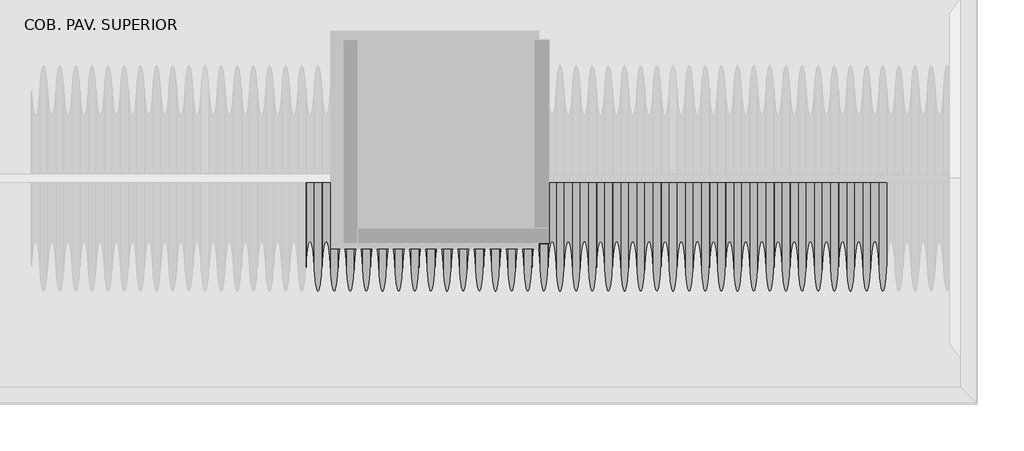
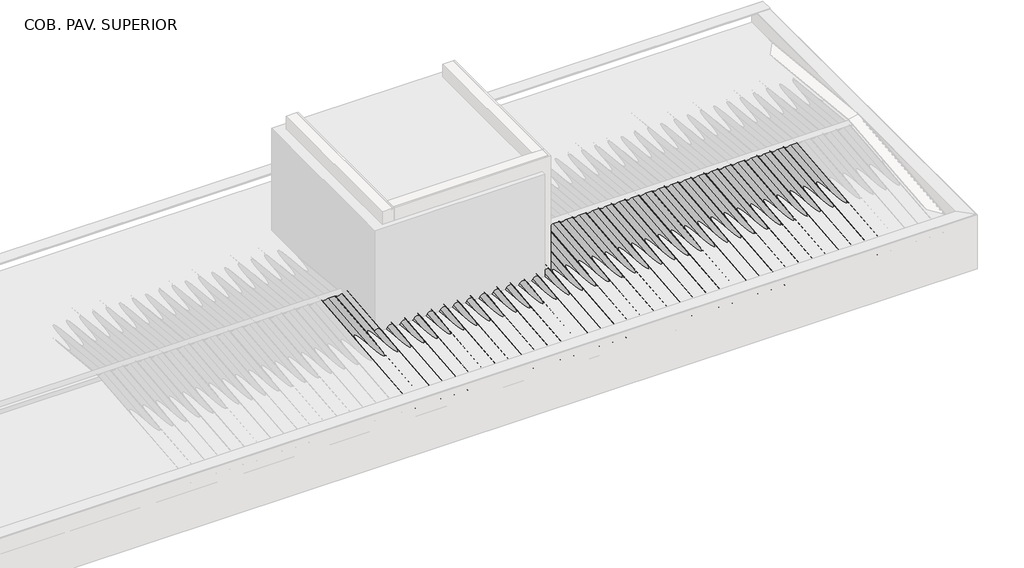
# One storey, part 6 of 8: 45 beams, 9 columns.
"""IFC4 building model written with IfcOpenShell, lengths in millimetres."""

import ifcopenshell
import ifcopenshell.guid

model = None  # the IFC model being written
_history = None  # IfcOwnerHistory: only IFC2X3 demands one
_inside = {}  # id of a spatial element -> (the spatial element, [elements in it])
_under = {}  # id of a project, library or spatial element -> (it, [spatial elements below it])
_declared = {}  # id of a project -> (the project, [libraries it declares])
_typed = {}  # id of a type object -> (the type object, [elements of that type])
_made_of = {}  # id of a material, layer set ... -> (it, [elements and type objects made of it])


def new_model(schema):
    """Start an empty IFC model of exactly this schema.

    Asked for "IFC4X3", IfcOpenShell would pick the latest addendum, in which some entities
    have other attributes; the version numbers below select the first issue.
    IFC2X3 requires an IfcOwnerHistory on every rooted entity: one is made here for all.
    """
    global model, _history
    if schema == "IFC4X3":
        model = ifcopenshell.file(schema_version=(4, 3, 0, 0))
    else:
        model = ifcopenshell.file(schema=schema)
    _inside.clear()
    _under.clear()
    _declared.clear()
    _typed.clear()
    _made_of.clear()
    _history = None
    if model.schema == "IFC2X3":
        org = make("IfcOrganization", Name="unknown")
        user = make(
            "IfcPersonAndOrganization",
            ThePerson=make("IfcPerson", FamilyName="unknown"),
            TheOrganization=org,
        )
        app = make(
            "IfcApplication",
            ApplicationDeveloper=org,
            Version="unknown",
            ApplicationFullName="unknown",
            ApplicationIdentifier="unknown",
        )
        _history = make(
            "IfcOwnerHistory",
            OwningUser=user,
            OwningApplication=app,
            ChangeAction="ADDED",
            CreationDate=0,
        )
    return model


def make(cls, **values):
    """One entity of the class cls with the attributes given. An attribute that is None is left unset."""
    return model.create_entity(
        cls, **{name: value for name, value in values.items() if value is not None}
    )


def rooted(cls, **values):
    """An entity with a GlobalId (a new one), such as an element, a storey or a relation."""
    return make(cls, GlobalId=ifcopenshell.guid.new(), OwnerHistory=_history, **values)


def si_unit(unit_type, name, prefix=None):
    """IfcSIUnit, for example si_unit("LENGTHUNIT", "METRE", prefix="MILLI")."""
    return make("IfcSIUnit", UnitType=unit_type, Prefix=prefix, Name=name)


def assignment(units):
    """IfcUnitAssignment: the units of a project."""
    return None if units is None else make("IfcUnitAssignment", Units=units)


def point(xyz):
    """IfcCartesianPoint."""
    return None if xyz is None else make("IfcCartesianPoint", Coordinates=xyz)


def direction(xyz):
    """IfcDirection."""
    return None if xyz is None else make("IfcDirection", DirectionRatios=xyz)


def frame(location, z_axis=None, x_axis=None):
    """IfcAxis2Placement3D, a coordinate frame: its origin and axes. An axis left out is left unset."""
    return make(
        "IfcAxis2Placement3D",
        Location=point(location),
        Axis=direction(z_axis),
        RefDirection=direction(x_axis),
    )


def frame_2d(location, x_axis=None):
    """IfcAxis2Placement2D, a coordinate frame in the plane: its origin and x axis."""
    return make(
        "IfcAxis2Placement2D", Location=point(location), RefDirection=direction(x_axis)
    )


def origin():
    """The frame at (0, 0, 0) with its axes left unset."""
    return frame((0.0, 0.0, 0.0))


def place(relative_to, where):
    """IfcLocalPlacement: puts the frame where relative to a parent placement (None: the world)."""
    return make(
        "IfcLocalPlacement", PlacementRelTo=relative_to, RelativePlacement=where
    )


def context(
    kind, dimensions, precision=None, world=None, true_north=None, identifier=None
):
    """IfcGeometricRepresentationContext, for example the 3D "Model" context."""
    return make(
        "IfcGeometricRepresentationContext",
        ContextIdentifier=identifier,
        ContextType=kind,
        CoordinateSpaceDimension=dimensions,
        Precision=precision,
        WorldCoordinateSystem=world,
        TrueNorth=true_north,
    )


def project(units=None, contexts=None):
    """IfcProject with its units and contexts."""
    return rooted(
        "IfcProject",
        Name="project",
        RepresentationContexts=contexts,
        UnitsInContext=assignment(units),
    )


def spatial(cls, under=None, at=None, **own):
    """A site, building, storey or space (cls), placed at a placement, below another one or the project."""
    s = rooted(cls, ObjectPlacement=at, **own)
    if under is not None:
        _under.setdefault(under.id(), (under, []))[1].append(s)
    return s


def polyline(points):
    """IfcPolyline through the points."""
    return make("IfcPolyline", Points=[point(p) for p in points])


def circle_curve(where, radius):
    """IfcCircle in the frame where."""
    return make("IfcCircle", Position=where, Radius=radius)


def trimmed(basis, trim1, trim2, sense, master):
    """IfcTrimmedCurve: the piece of a basis curve between two trims."""
    return make(
        "IfcTrimmedCurve",
        BasisCurve=basis,
        Trim1=trim1,
        Trim2=trim2,
        SenseAgreement=sense,
        MasterRepresentation=master,
    )


def segment(curve, same_sense, transition):
    """IfcCompositeCurveSegment."""
    return make(
        "IfcCompositeCurveSegment",
        Transition=transition,
        SameSense=same_sense,
        ParentCurve=curve,
    )


def composite_curve(segments, self_intersect=None):
    """IfcCompositeCurve: segments joined end to end."""
    return make("IfcCompositeCurve", Segments=segments, SelfIntersect=self_intersect)


def outline(outer, holes=None, kind="AREA"):
    """IfcArbitraryClosedProfileDef: a profile drawn as a closed curve; with holes, ...WithVoids."""
    if holes is None:
        return make("IfcArbitraryClosedProfileDef", ProfileType=kind, OuterCurve=outer)
    return make(
        "IfcArbitraryProfileDefWithVoids",
        ProfileType=kind,
        OuterCurve=outer,
        InnerCurves=holes,
    )


def extrude(swept, where, along, depth):
    """IfcExtrudedAreaSolid: the profile swept, set in the frame where, extruded along a direction by depth."""
    return make(
        "IfcExtrudedAreaSolid",
        SweptArea=swept,
        Position=where,
        ExtrudedDirection=direction(along),
        Depth=depth,
    )


def shape(context_of_items, identifier, shape_type, items):
    """IfcShapeRepresentation: the items that make up one representation, for example the "Body"."""
    return make(
        "IfcShapeRepresentation",
        ContextOfItems=context_of_items,
        RepresentationIdentifier=identifier,
        RepresentationType=shape_type,
        Items=items,
    )


def source(mapping_origin, context_of_items, identifier, shape_type, items):
    """IfcRepresentationMap: a shape defined once, which mapped items show again and again."""
    return make(
        "IfcRepresentationMap",
        MappingOrigin=mapping_origin,
        MappedRepresentation=shape(context_of_items, identifier, shape_type, items),
    )


def transform(
    local_origin,
    x_axis=None,
    y_axis=None,
    z_axis=None,
    scale=None,
    scale2=None,
    scale3=None,
    uniform=True,
):
    """IfcCartesianTransformationOperator3D, or its non-uniform kind. x_axis, y_axis, z_axis: its Axis1, 2, 3."""
    if uniform:
        return make(
            "IfcCartesianTransformationOperator3D",
            Axis1=direction(x_axis),
            Axis2=direction(y_axis),
            LocalOrigin=point(local_origin),
            Scale=scale,
            Axis3=direction(z_axis),
        )
    return make(
        "IfcCartesianTransformationOperator3DnonUniform",
        Axis1=direction(x_axis),
        Axis2=direction(y_axis),
        LocalOrigin=point(local_origin),
        Scale=scale,
        Axis3=direction(z_axis),
        Scale2=scale2,
        Scale3=scale3,
    )


def mapped(mapping_source, mapping_target):
    """IfcMappedItem: shows the shape of a source again, moved by a transform."""
    return make(
        "IfcMappedItem", MappingSource=mapping_source, MappingTarget=mapping_target
    )


def made_of(thing, what):
    """Note that an element or type object is made of a material, layer set ...; save() writes the relation."""
    if what is not None:
        _made_of.setdefault(what.id(), (what, []))[1].append(thing)
    return thing


def element(
    cls,
    number,
    at=None,
    inside=None,
    cuts=None,
    type_object=None,
    material=None,
    context=None,
    identifier="Body",
    shape_type=None,
    held_by="IfcProductDefinitionShape",
    body=None,
    shapes=None,
    **own,
):
    """One element of the class cls, such as IfcWall. Its Tag is "e" and its number.

    at: its placement. inside: the storey or other place that contains it. cuts: it is an
    opening in that element (IfcRelVoidsElement). A single representation is given by context,
    identifier, shape_type and body (its items); several are given by shapes. held_by: the class
    of the entity that holds the representations. save() writes the other relations.
    """
    e = rooted(cls, Tag="e%d" % number, ObjectPlacement=at, **own)
    if body is not None:
        shapes = [shape(context, identifier, shape_type, body)]
    if shapes is not None:
        e.Representation = make(held_by, Representations=shapes)
    if inside is not None:
        _inside.setdefault(inside.id(), (inside, []))[1].append(e)
    if cuts is not None:
        rooted(
            "IfcRelVoidsElement", RelatingBuildingElement=cuts, RelatedOpeningElement=e
        )
    if type_object is not None:
        _typed.setdefault(type_object.id(), (type_object, []))[1].append(e)
    return made_of(e, material)


def aggregate(whole, parts):
    """IfcRelAggregates: a whole, such as a stair, and the parts it consists of."""
    return rooted("IfcRelAggregates", RelatingObject=whole, RelatedObjects=parts)


def save(model, path):
    """Write the relations noted so far, then the file.

    IfcRelAggregates (storeys below a building ...), IfcRelContainedInSpatialStructure (elements
    in a storey), IfcRelDefinesByType, IfcRelAssociatesMaterial and IfcRelDeclares: one each for
    every whole, place, type object, material and project.
    """
    for whole, parts in _under.values():
        aggregate(whole, parts)
    for where, things in _inside.values():
        rooted(
            "IfcRelContainedInSpatialStructure",
            RelatedElements=things,
            RelatingStructure=where,
        )
    for kind, things in _typed.values():
        rooted("IfcRelDefinesByType", RelatedObjects=things, RelatingType=kind)
    for what, things in _made_of.values():
        rooted("IfcRelAssociatesMaterial", RelatedObjects=things, RelatingMaterial=what)
    for by, libraries in _declared.values():
        rooted("IfcRelDeclares", RelatingContext=by, RelatedDefinitions=libraries)
    model.write(path)


def beam_fe4ddbad(model_context):
    return source(origin(), model_context, "Body", "SweptSolid", [
        extrude(outline(polyline([(998.8971968, 30.0), (998.8971968, -30.0), (-998.8971974, -30.0), (-998.8971974, 30.0), (998.8971968, 30.0)])), frame((0.0, 0.0, -60.0), z_axis=(0.0, 0.0, 1.0), x_axis=(1.0, 0.0, 0.0)), (0.0, 0.0, 1.0), 120.0),
    ])


def beam_c6e4bd39(model_context):
    return source(origin(), model_context, "Body", "SweptSolid", [
        extrude(outline(polyline([(789.5373463, 30.0), (789.5373463, -30.0), (-789.5373463, -30.0), (-789.5373463, 30.0), (789.5373463, 30.0)])), frame((0.0, 0.0, -60.0), z_axis=(0.0, 0.0, 1.0), x_axis=(1.0, 0.0, 0.0)), (0.0, 0.0, 1.0), 120.0),
    ])


def telha_ondulada_fibrocimento_69359d52(model_context):
    return source(origin(), model_context, "Body", "SweptSolid", [
        extrude(outline(composite_curve([segment(trimmed(circle_curve(frame_2d((68.3970135, 71.7939461)), 66.7939461), [point((8.3970135, 42.4437972))], [point((128.3970135, 42.4437972))], True, "CARTESIAN"), True, "CONTINUOUS"), segment(polyline([(128.3970135, 42.4437972), (132.8884385, 40.2467307)]), True, "CONTINUOUS"), segment(trimmed(circle_curve(frame_2d((68.3970135, 71.7939461)), 71.7939461), [point((132.8884385, 40.2467307))], [point((3.9055884, 40.2467307))], False, "CARTESIAN"), True, "CONTINUOUS"), segment(trimmed(circle_curve(frame_2d((-51.6029865, 13.0936483)), 61.7939461), [point((3.9055884, 40.2467307))], [point((-107.1115615, 40.2467307))], True, "CARTESIAN"), True, "CONTINUOUS"), segment(polyline([(-107.1115615, 40.2467307), (-111.6029865, 42.4437972)]), True, "CONTINUOUS"), segment(trimmed(circle_curve(frame_2d((-51.6029865, 13.0936483)), 66.7939461), [point((-111.6029865, 42.4437972))], [point((8.3970135, 42.4437972))], False, "CARTESIAN"), True, "CONTINUOUS")], self_intersect=False)), frame((-1038.2805783, 0.0, 0.0), z_axis=(1.0, 0.0, 0.0), x_axis=(0.0, 1.0, 0.0)), (0.0, 0.0, 1.0), 2076.5611566),
    ])


def column_6c15bf79(model_context):
    return source(origin(), model_context, "Body", "SweptSolid", [
        extrude(outline(polyline([(30.0, 80.0), (30.0, -80.0), (-30.0, -80.0), (-30.0, 80.0), (30.0, 80.0)])), frame((0.0, 0.0, 6710.0), z_axis=(0.0, 0.0, 1.0), x_axis=(1.0, 0.0, 0.0)), (0.0, 0.0, 1.0), 467.5),
    ])


def column_42eef9f8(model_context):
    return source(origin(), model_context, "Body", "SweptSolid", [
        extrude(outline(polyline([(30.0, 80.0), (30.0, -80.0), (-30.0, -80.0), (-30.0, 80.0), (30.0, 80.0)])), frame((0.0, 0.0, 6710.0), z_axis=(0.0, 0.0, 1.0), x_axis=(1.0, 0.0, 0.0)), (0.0, 0.0, 1.0), 227.1),
    ])


model = new_model("IFC4")

# Units and contexts
model_context = context("Model", 3, world=origin())
ifc_project = project(units=[si_unit("LENGTHUNIT", "METRE", prefix="MILLI")], contexts=[model_context])

# Site, building, storey
site = spatial("IfcSite", under=ifc_project)
building = spatial("IfcBuilding", under=site)
storey = spatial("IfcBuildingStorey", under=building, Name="COB. PAV. SUPERIOR", Elevation=6650.0)

# Beams
placement = place(None, origin())
beam_shape = beam_fe4ddbad(model_context)
element("IfcBeam", 1, ObjectType="Madeira de lei : Berço 6x12cm", at=placement, inside=storey, context=model_context, shape_type="MappedRepresentation", body=[
    mapped(beam_shape, transform((248.5822594, -9189.768869, 6680.0), x_axis=(1.0, 0.0, 0.0), y_axis=(0.0, 0.0, -1.0), z_axis=(0.0, 1.0, 0.0))),
])
element("IfcBeam", 2, ObjectType="Madeira de lei : Berço 6x12cm", at=placement, inside=storey, context=model_context, shape_type="MappedRepresentation", body=[
    mapped(beam_shape, transform((2246.3766542, -9189.768869, 6680.0), x_axis=(1.0, 0.0, 0.0), y_axis=(0.0, 0.0, -1.0), z_axis=(0.0, 1.0, 0.0))),
])
element("IfcBeam", 3, ObjectType="Madeira de lei : Berço 6x12cm", at=placement, inside=storey, context=model_context, shape_type="MappedRepresentation", body=[
    mapped(beam_shape, transform((4244.171049, -9189.768869, 6680.0), x_axis=(1.0, 0.0, 0.0), y_axis=(0.0, 0.0, -1.0), z_axis=(0.0, 1.0, 0.0))),
])
element("IfcBeam", 4, ObjectType="Madeira de lei : Berço 6x12cm", at=placement, inside=storey, context=model_context, shape_type="MappedRepresentation", body=[
    mapped(beam_shape, transform((6241.9654438, -9189.768869, 6680.0), x_axis=(1.0, 0.0, 0.0), y_axis=(0.0, 0.0, -1.0), z_axis=(0.0, 1.0, 0.0))),
])
element("IfcBeam", 5, ObjectType="Madeira de lei : Berço 6x12cm", at=placement, inside=storey, context=model_context, shape_type="MappedRepresentation", body=[
    mapped(beam_shape, transform((8239.7598386, -9189.768869, 6680.0), x_axis=(1.0, 0.0, 0.0), y_axis=(0.0, 0.0, -1.0), z_axis=(0.0, 1.0, 0.0))),
])
element("IfcBeam", 6, ObjectType="Madeira de lei : Berço 6x12cm", at=placement, inside=storey, context=model_context, shape_type="MappedRepresentation", body=[
    mapped(beam_shape, transform((4244.171049, -10631.818869, 6680.0), x_axis=(1.0, 0.0, 0.0), y_axis=(0.0, 0.0, -1.0), z_axis=(0.0, 1.0, 0.0))),
])
element("IfcBeam", 7, ObjectType="Madeira de lei : Berço 6x12cm", at=placement, inside=storey, context=model_context, shape_type="MappedRepresentation", body=[
    mapped(beam_shape, transform((6241.9654438, -10631.818869, 6680.0), x_axis=(1.0, 0.0, 0.0), y_axis=(0.0, 0.0, -1.0), z_axis=(0.0, 1.0, 0.0))),
])
element("IfcBeam", 8, ObjectType="Madeira de lei : Berço 6x12cm", at=placement, inside=storey, context=model_context, shape_type="MappedRepresentation", body=[
    mapped(beam_shape, transform((8239.7598386, -10631.818869, 6680.0), x_axis=(1.0, 0.0, 0.0), y_axis=(0.0, 0.0, -1.0), z_axis=(0.0, 1.0, 0.0))),
])
beam_2_shape = beam_c6e4bd39(model_context)
element("IfcBeam", 9, ObjectType="Madeira de lei : Berço 6x12cm", at=placement, inside=storey, context=model_context, shape_type="MappedRepresentation", body=[
    mapped(beam_2_shape, transform((10028.1943824, -10631.818869, 6680.0), x_axis=(1.0, 0.0, 0.0), y_axis=(0.0, 0.0, -1.0), z_axis=(0.0, 1.0, 0.0))),
])
element("IfcBeam", 10, ObjectType="Telha Ondulada : Fibrocimento", at=placement, inside=storey, context=model_context, shape_type="SweptSolid", body=[
    extrude(outline(composite_curve([segment(trimmed(circle_curve(frame_2d((0.0, 66.7939461)), 66.7939461), [point((29.3501489, 6.7939461))], [point((29.3501489, 126.7939461))], True, "CARTESIAN"), True, "CONTINUOUS"), segment(polyline([(29.3501489, 126.7939461), (31.5472154, 131.2853711)]), True, "CONTINUOUS"), segment(trimmed(circle_curve(frame_2d((0.0, 66.7939461)), 71.7939461), [point((31.5472154, 131.2853711))], [point((31.5472154, 2.3025211))], False, "CARTESIAN"), True, "CONTINUOUS"), segment(trimmed(circle_curve(frame_2d((58.7002978, -53.2060539)), 61.7939461), [point((31.5472154, 2.3025211))], [point((31.5472154, -108.7146289))], True, "CARTESIAN"), True, "CONTINUOUS"), segment(polyline([(31.5472154, -108.7146289), (29.3501489, -113.2060539)]), True, "CONTINUOUS"), segment(trimmed(circle_curve(frame_2d((58.7002978, -53.2060539)), 66.7939461), [point((29.3501489, -113.2060539))], [point((29.3501489, 6.7939461))], False, "CARTESIAN"), True, "CONTINUOUS")], self_intersect=False)), frame((994.7156257, -10831.9594023, 7106.8215886), z_axis=(0.0, 0.9950371902099894, 0.09950371902099749), x_axis=(0.0, 0.09950371902099749, -0.9950371902099894)), (0.0, 0.0, 1.0), 3060.4439799),
])
element("IfcBeam", 11, ObjectType="Telha Ondulada : Fibrocimento", at=placement, inside=storey, context=model_context, shape_type="SweptSolid", body=[
    extrude(outline(composite_curve([segment(trimmed(circle_curve(frame_2d((0.0, 66.7939461)), 66.7939461), [point((29.3501489, 6.7939461))], [point((29.3501489, 126.7939461))], True, "CARTESIAN"), True, "CONTINUOUS"), segment(polyline([(29.3501489, 126.7939461), (31.5472154, 131.2853711)]), True, "CONTINUOUS"), segment(trimmed(circle_curve(frame_2d((0.0, 66.7939461)), 71.7939461), [point((31.5472154, 131.2853711))], [point((31.5472154, 2.3025211))], False, "CARTESIAN"), True, "CONTINUOUS"), segment(trimmed(circle_curve(frame_2d((58.7002978, -53.2060539)), 61.7939461), [point((31.5472154, 2.3025211))], [point((31.5472154, -108.7146289))], True, "CARTESIAN"), True, "CONTINUOUS"), segment(polyline([(31.5472154, -108.7146289), (29.3501489, -113.2060539)]), True, "CONTINUOUS"), segment(trimmed(circle_curve(frame_2d((58.7002978, -53.2060539)), 66.7939461), [point((29.3501489, -113.2060539))], [point((29.3501489, 6.7939461))], False, "CARTESIAN"), True, "CONTINUOUS")], self_intersect=False)), frame((1239.2156257, -10831.9594023, 7106.8215886), z_axis=(0.0, 0.9950371902099894, 0.09950371902099749), x_axis=(0.0, 0.09950371902099749, -0.9950371902099894)), (0.0, 0.0, 1.0), 3060.4439799),
])
element("IfcBeam", 12, ObjectType="Telha Ondulada : Fibrocimento", at=placement, inside=storey, context=model_context, shape_type="SweptSolid", body=[
    extrude(outline(composite_curve([segment(trimmed(circle_curve(frame_2d((0.0, 66.7939461)), 66.7939461), [point((29.3501489, 6.7939461))], [point((29.3501489, 126.7939461))], True, "CARTESIAN"), True, "CONTINUOUS"), segment(polyline([(29.3501489, 126.7939461), (31.5472154, 131.2853711)]), True, "CONTINUOUS"), segment(trimmed(circle_curve(frame_2d((0.0, 66.7939461)), 71.7939461), [point((31.5472154, 131.2853711))], [point((31.5472154, 2.3025211))], False, "CARTESIAN"), True, "CONTINUOUS"), segment(trimmed(circle_curve(frame_2d((58.7002978, -53.2060539)), 61.7939461), [point((31.5472154, 2.3025211))], [point((31.5472154, -108.7146289))], True, "CARTESIAN"), True, "CONTINUOUS"), segment(polyline([(31.5472154, -108.7146289), (29.3501489, -113.2060539)]), True, "CONTINUOUS"), segment(trimmed(circle_curve(frame_2d((58.7002978, -53.2060539)), 66.7939461), [point((29.3501489, -113.2060539))], [point((29.3501489, 6.7939461))], False, "CARTESIAN"), True, "CONTINUOUS")], self_intersect=False)), frame((4662.2156257, -10831.9594023, 7106.8215886), z_axis=(0.0, 0.9950371902099894, 0.09950371902099749), x_axis=(0.0, 0.09950371902099749, -0.9950371902099894)), (0.0, 0.0, 1.0), 3060.4439799),
])
element("IfcBeam", 13, ObjectType="Telha Ondulada : Fibrocimento", at=placement, inside=storey, context=model_context, shape_type="SweptSolid", body=[
    extrude(outline(composite_curve([segment(trimmed(circle_curve(frame_2d((0.0, 66.7939461)), 66.7939461), [point((29.3501489, 6.7939461))], [point((29.3501489, 126.7939461))], True, "CARTESIAN"), True, "CONTINUOUS"), segment(polyline([(29.3501489, 126.7939461), (31.5472154, 131.2853711)]), True, "CONTINUOUS"), segment(trimmed(circle_curve(frame_2d((0.0, 66.7939461)), 71.7939461), [point((31.5472154, 131.2853711))], [point((31.5472154, 2.3025211))], False, "CARTESIAN"), True, "CONTINUOUS"), segment(trimmed(circle_curve(frame_2d((58.7002978, -53.2060539)), 61.7939461), [point((31.5472154, 2.3025211))], [point((31.5472154, -108.7146289))], True, "CARTESIAN"), True, "CONTINUOUS"), segment(polyline([(31.5472154, -108.7146289), (29.3501489, -113.2060539)]), True, "CONTINUOUS"), segment(trimmed(circle_curve(frame_2d((58.7002978, -53.2060539)), 66.7939461), [point((29.3501489, -113.2060539))], [point((29.3501489, 6.7939461))], False, "CARTESIAN"), True, "CONTINUOUS")], self_intersect=False)), frame((4906.7156257, -10831.9594023, 7106.8215886), z_axis=(0.0, 0.9950371902099894, 0.09950371902099749), x_axis=(0.0, 0.09950371902099749, -0.9950371902099894)), (0.0, 0.0, 1.0), 3060.4439799),
])
element("IfcBeam", 14, ObjectType="Telha Ondulada : Fibrocimento", at=placement, inside=storey, context=model_context, shape_type="SweptSolid", body=[
    extrude(outline(composite_curve([segment(trimmed(circle_curve(frame_2d((0.0, 66.7939461)), 66.7939461), [point((29.3501489, 6.7939461))], [point((29.3501489, 126.7939461))], True, "CARTESIAN"), True, "CONTINUOUS"), segment(polyline([(29.3501489, 126.7939461), (31.5472154, 131.2853711)]), True, "CONTINUOUS"), segment(trimmed(circle_curve(frame_2d((0.0, 66.7939461)), 71.7939461), [point((31.5472154, 131.2853711))], [point((31.5472154, 2.3025211))], False, "CARTESIAN"), True, "CONTINUOUS"), segment(trimmed(circle_curve(frame_2d((58.7002978, -53.2060539)), 61.7939461), [point((31.5472154, 2.3025211))], [point((31.5472154, -108.7146289))], True, "CARTESIAN"), True, "CONTINUOUS"), segment(polyline([(31.5472154, -108.7146289), (29.3501489, -113.2060539)]), True, "CONTINUOUS"), segment(trimmed(circle_curve(frame_2d((58.7002978, -53.2060539)), 66.7939461), [point((29.3501489, -113.2060539))], [point((29.3501489, 6.7939461))], False, "CARTESIAN"), True, "CONTINUOUS")], self_intersect=False)), frame((5151.2156257, -10831.9594023, 7106.8215886), z_axis=(0.0, 0.9950371902099894, 0.09950371902099749), x_axis=(0.0, 0.09950371902099749, -0.9950371902099894)), (0.0, 0.0, 1.0), 3060.4439799),
])
element("IfcBeam", 15, ObjectType="Telha Ondulada : Fibrocimento", at=placement, inside=storey, context=model_context, shape_type="SweptSolid", body=[
    extrude(outline(composite_curve([segment(trimmed(circle_curve(frame_2d((0.0, 66.7939461)), 66.7939461), [point((29.3501489, 6.7939461))], [point((29.3501489, 126.7939461))], True, "CARTESIAN"), True, "CONTINUOUS"), segment(polyline([(29.3501489, 126.7939461), (31.5472154, 131.2853711)]), True, "CONTINUOUS"), segment(trimmed(circle_curve(frame_2d((0.0, 66.7939461)), 71.7939461), [point((31.5472154, 131.2853711))], [point((31.5472154, 2.3025211))], False, "CARTESIAN"), True, "CONTINUOUS"), segment(trimmed(circle_curve(frame_2d((58.7002978, -53.2060539)), 61.7939461), [point((31.5472154, 2.3025211))], [point((31.5472154, -108.7146289))], True, "CARTESIAN"), True, "CONTINUOUS"), segment(polyline([(31.5472154, -108.7146289), (29.3501489, -113.2060539)]), True, "CONTINUOUS"), segment(trimmed(circle_curve(frame_2d((58.7002978, -53.2060539)), 66.7939461), [point((29.3501489, -113.2060539))], [point((29.3501489, 6.7939461))], False, "CARTESIAN"), True, "CONTINUOUS")], self_intersect=False)), frame((5395.7156257, -10831.9594023, 7106.8215886), z_axis=(0.0, 0.9950371902099894, 0.09950371902099749), x_axis=(0.0, 0.09950371902099749, -0.9950371902099894)), (0.0, 0.0, 1.0), 3060.4439799),
])
element("IfcBeam", 16, ObjectType="Telha Ondulada : Fibrocimento", at=placement, inside=storey, context=model_context, shape_type="SweptSolid", body=[
    extrude(outline(composite_curve([segment(trimmed(circle_curve(frame_2d((0.0, 66.7939461)), 66.7939461), [point((29.3501489, 6.7939461))], [point((29.3501489, 126.7939461))], True, "CARTESIAN"), True, "CONTINUOUS"), segment(polyline([(29.3501489, 126.7939461), (31.5472154, 131.2853711)]), True, "CONTINUOUS"), segment(trimmed(circle_curve(frame_2d((0.0, 66.7939461)), 71.7939461), [point((31.5472154, 131.2853711))], [point((31.5472154, 2.3025211))], False, "CARTESIAN"), True, "CONTINUOUS"), segment(trimmed(circle_curve(frame_2d((58.7002978, -53.2060539)), 61.7939461), [point((31.5472154, 2.3025211))], [point((31.5472154, -108.7146289))], True, "CARTESIAN"), True, "CONTINUOUS"), segment(polyline([(31.5472154, -108.7146289), (29.3501489, -113.2060539)]), True, "CONTINUOUS"), segment(trimmed(circle_curve(frame_2d((58.7002978, -53.2060539)), 66.7939461), [point((29.3501489, -113.2060539))], [point((29.3501489, 6.7939461))], False, "CARTESIAN"), True, "CONTINUOUS")], self_intersect=False)), frame((5640.2156257, -10831.9594023, 7106.8215886), z_axis=(0.0, 0.9950371902099894, 0.09950371902099749), x_axis=(0.0, 0.09950371902099749, -0.9950371902099894)), (0.0, 0.0, 1.0), 3060.4439799),
])
element("IfcBeam", 17, ObjectType="Telha Ondulada : Fibrocimento", at=placement, inside=storey, context=model_context, shape_type="SweptSolid", body=[
    extrude(outline(composite_curve([segment(trimmed(circle_curve(frame_2d((0.0, 66.7939461)), 66.7939461), [point((29.3501489, 6.7939461))], [point((29.3501489, 126.7939461))], True, "CARTESIAN"), True, "CONTINUOUS"), segment(polyline([(29.3501489, 126.7939461), (31.5472154, 131.2853711)]), True, "CONTINUOUS"), segment(trimmed(circle_curve(frame_2d((0.0, 66.7939461)), 71.7939461), [point((31.5472154, 131.2853711))], [point((31.5472154, 2.3025211))], False, "CARTESIAN"), True, "CONTINUOUS"), segment(trimmed(circle_curve(frame_2d((58.7002978, -53.2060539)), 61.7939461), [point((31.5472154, 2.3025211))], [point((31.5472154, -108.7146289))], True, "CARTESIAN"), True, "CONTINUOUS"), segment(polyline([(31.5472154, -108.7146289), (29.3501489, -113.2060539)]), True, "CONTINUOUS"), segment(trimmed(circle_curve(frame_2d((58.7002978, -53.2060539)), 66.7939461), [point((29.3501489, -113.2060539))], [point((29.3501489, 6.7939461))], False, "CARTESIAN"), True, "CONTINUOUS")], self_intersect=False)), frame((5884.7156257, -10831.9594023, 7106.8215886), z_axis=(0.0, 0.9950371902099894, 0.09950371902099749), x_axis=(0.0, 0.09950371902099749, -0.9950371902099894)), (0.0, 0.0, 1.0), 3060.4439799),
])
element("IfcBeam", 18, ObjectType="Telha Ondulada : Fibrocimento", at=placement, inside=storey, context=model_context, shape_type="SweptSolid", body=[
    extrude(outline(composite_curve([segment(trimmed(circle_curve(frame_2d((0.0, 66.7939461)), 66.7939461), [point((29.3501489, 6.7939461))], [point((29.3501489, 126.7939461))], True, "CARTESIAN"), True, "CONTINUOUS"), segment(polyline([(29.3501489, 126.7939461), (31.5472154, 131.2853711)]), True, "CONTINUOUS"), segment(trimmed(circle_curve(frame_2d((0.0, 66.7939461)), 71.7939461), [point((31.5472154, 131.2853711))], [point((31.5472154, 2.3025211))], False, "CARTESIAN"), True, "CONTINUOUS"), segment(trimmed(circle_curve(frame_2d((58.7002978, -53.2060539)), 61.7939461), [point((31.5472154, 2.3025211))], [point((31.5472154, -108.7146289))], True, "CARTESIAN"), True, "CONTINUOUS"), segment(polyline([(31.5472154, -108.7146289), (29.3501489, -113.2060539)]), True, "CONTINUOUS"), segment(trimmed(circle_curve(frame_2d((58.7002978, -53.2060539)), 66.7939461), [point((29.3501489, -113.2060539))], [point((29.3501489, 6.7939461))], False, "CARTESIAN"), True, "CONTINUOUS")], self_intersect=False)), frame((6129.2156257, -10831.9594023, 7106.8215886), z_axis=(0.0, 0.9950371902099894, 0.09950371902099749), x_axis=(0.0, 0.09950371902099749, -0.9950371902099894)), (0.0, 0.0, 1.0), 3060.4439799),
])
element("IfcBeam", 19, ObjectType="Telha Ondulada : Fibrocimento", at=placement, inside=storey, context=model_context, shape_type="SweptSolid", body=[
    extrude(outline(composite_curve([segment(trimmed(circle_curve(frame_2d((0.0, 66.7939461)), 66.7939461), [point((29.3501489, 6.7939461))], [point((29.3501489, 126.7939461))], True, "CARTESIAN"), True, "CONTINUOUS"), segment(polyline([(29.3501489, 126.7939461), (31.5472154, 131.2853711)]), True, "CONTINUOUS"), segment(trimmed(circle_curve(frame_2d((0.0, 66.7939461)), 71.7939461), [point((31.5472154, 131.2853711))], [point((31.5472154, 2.3025211))], False, "CARTESIAN"), True, "CONTINUOUS"), segment(trimmed(circle_curve(frame_2d((58.7002978, -53.2060539)), 61.7939461), [point((31.5472154, 2.3025211))], [point((31.5472154, -108.7146289))], True, "CARTESIAN"), True, "CONTINUOUS"), segment(polyline([(31.5472154, -108.7146289), (29.3501489, -113.2060539)]), True, "CONTINUOUS"), segment(trimmed(circle_curve(frame_2d((58.7002978, -53.2060539)), 66.7939461), [point((29.3501489, -113.2060539))], [point((29.3501489, 6.7939461))], False, "CARTESIAN"), True, "CONTINUOUS")], self_intersect=False)), frame((6373.7156257, -10831.9594023, 7106.8215886), z_axis=(0.0, 0.9950371902099894, 0.09950371902099749), x_axis=(0.0, 0.09950371902099749, -0.9950371902099894)), (0.0, 0.0, 1.0), 3060.4439799),
])
element("IfcBeam", 20, ObjectType="Telha Ondulada : Fibrocimento", at=placement, inside=storey, context=model_context, shape_type="SweptSolid", body=[
    extrude(outline(composite_curve([segment(trimmed(circle_curve(frame_2d((0.0, 66.7939461)), 66.7939461), [point((29.3501489, 6.7939461))], [point((29.3501489, 126.7939461))], True, "CARTESIAN"), True, "CONTINUOUS"), segment(polyline([(29.3501489, 126.7939461), (31.5472154, 131.2853711)]), True, "CONTINUOUS"), segment(trimmed(circle_curve(frame_2d((0.0, 66.7939461)), 71.7939461), [point((31.5472154, 131.2853711))], [point((31.5472154, 2.3025211))], False, "CARTESIAN"), True, "CONTINUOUS"), segment(trimmed(circle_curve(frame_2d((58.7002978, -53.2060539)), 61.7939461), [point((31.5472154, 2.3025211))], [point((31.5472154, -108.7146289))], True, "CARTESIAN"), True, "CONTINUOUS"), segment(polyline([(31.5472154, -108.7146289), (29.3501489, -113.2060539)]), True, "CONTINUOUS"), segment(trimmed(circle_curve(frame_2d((58.7002978, -53.2060539)), 66.7939461), [point((29.3501489, -113.2060539))], [point((29.3501489, 6.7939461))], False, "CARTESIAN"), True, "CONTINUOUS")], self_intersect=False)), frame((6618.2156257, -10831.9594023, 7106.8215886), z_axis=(0.0, 0.9950371902099894, 0.09950371902099749), x_axis=(0.0, 0.09950371902099749, -0.9950371902099894)), (0.0, 0.0, 1.0), 3060.4439799),
])
element("IfcBeam", 21, ObjectType="Telha Ondulada : Fibrocimento", at=placement, inside=storey, context=model_context, shape_type="SweptSolid", body=[
    extrude(outline(composite_curve([segment(trimmed(circle_curve(frame_2d((0.0, 66.7939461)), 66.7939461), [point((29.3501489, 6.7939461))], [point((29.3501489, 126.7939461))], True, "CARTESIAN"), True, "CONTINUOUS"), segment(polyline([(29.3501489, 126.7939461), (31.5472154, 131.2853711)]), True, "CONTINUOUS"), segment(trimmed(circle_curve(frame_2d((0.0, 66.7939461)), 71.7939461), [point((31.5472154, 131.2853711))], [point((31.5472154, 2.3025211))], False, "CARTESIAN"), True, "CONTINUOUS"), segment(trimmed(circle_curve(frame_2d((58.7002978, -53.2060539)), 61.7939461), [point((31.5472154, 2.3025211))], [point((31.5472154, -108.7146289))], True, "CARTESIAN"), True, "CONTINUOUS"), segment(polyline([(31.5472154, -108.7146289), (29.3501489, -113.2060539)]), True, "CONTINUOUS"), segment(trimmed(circle_curve(frame_2d((58.7002978, -53.2060539)), 66.7939461), [point((29.3501489, -113.2060539))], [point((29.3501489, 6.7939461))], False, "CARTESIAN"), True, "CONTINUOUS")], self_intersect=False)), frame((6862.7156257, -10831.9594023, 7106.8215886), z_axis=(0.0, 0.9950371902099894, 0.09950371902099749), x_axis=(0.0, 0.09950371902099749, -0.9950371902099894)), (0.0, 0.0, 1.0), 3060.4439799),
])
element("IfcBeam", 22, ObjectType="Telha Ondulada : Fibrocimento", at=placement, inside=storey, context=model_context, shape_type="SweptSolid", body=[
    extrude(outline(composite_curve([segment(trimmed(circle_curve(frame_2d((0.0, 66.7939461)), 66.7939461), [point((29.3501489, 6.7939461))], [point((29.3501489, 126.7939461))], True, "CARTESIAN"), True, "CONTINUOUS"), segment(polyline([(29.3501489, 126.7939461), (31.5472154, 131.2853711)]), True, "CONTINUOUS"), segment(trimmed(circle_curve(frame_2d((0.0, 66.7939461)), 71.7939461), [point((31.5472154, 131.2853711))], [point((31.5472154, 2.3025211))], False, "CARTESIAN"), True, "CONTINUOUS"), segment(trimmed(circle_curve(frame_2d((58.7002978, -53.2060539)), 61.7939461), [point((31.5472154, 2.3025211))], [point((31.5472154, -108.7146289))], True, "CARTESIAN"), True, "CONTINUOUS"), segment(polyline([(31.5472154, -108.7146289), (29.3501489, -113.2060539)]), True, "CONTINUOUS"), segment(trimmed(circle_curve(frame_2d((58.7002978, -53.2060539)), 66.7939461), [point((29.3501489, -113.2060539))], [point((29.3501489, 6.7939461))], False, "CARTESIAN"), True, "CONTINUOUS")], self_intersect=False)), frame((7107.2156257, -10831.9594023, 7106.8215886), z_axis=(0.0, 0.9950371902099894, 0.09950371902099749), x_axis=(0.0, 0.09950371902099749, -0.9950371902099894)), (0.0, 0.0, 1.0), 3060.4439799),
])
element("IfcBeam", 23, ObjectType="Telha Ondulada : Fibrocimento", at=placement, inside=storey, context=model_context, shape_type="SweptSolid", body=[
    extrude(outline(composite_curve([segment(trimmed(circle_curve(frame_2d((0.0, 66.7939461)), 66.7939461), [point((29.3501489, 6.7939461))], [point((29.3501489, 126.7939461))], True, "CARTESIAN"), True, "CONTINUOUS"), segment(polyline([(29.3501489, 126.7939461), (31.5472154, 131.2853711)]), True, "CONTINUOUS"), segment(trimmed(circle_curve(frame_2d((0.0, 66.7939461)), 71.7939461), [point((31.5472154, 131.2853711))], [point((31.5472154, 2.3025211))], False, "CARTESIAN"), True, "CONTINUOUS"), segment(trimmed(circle_curve(frame_2d((58.7002978, -53.2060539)), 61.7939461), [point((31.5472154, 2.3025211))], [point((31.5472154, -108.7146289))], True, "CARTESIAN"), True, "CONTINUOUS"), segment(polyline([(31.5472154, -108.7146289), (29.3501489, -113.2060539)]), True, "CONTINUOUS"), segment(trimmed(circle_curve(frame_2d((58.7002978, -53.2060539)), 66.7939461), [point((29.3501489, -113.2060539))], [point((29.3501489, 6.7939461))], False, "CARTESIAN"), True, "CONTINUOUS")], self_intersect=False)), frame((7351.7156257, -10831.9594023, 7106.8215886), z_axis=(0.0, 0.9950371902099894, 0.09950371902099749), x_axis=(0.0, 0.09950371902099749, -0.9950371902099894)), (0.0, 0.0, 1.0), 3060.4439799),
])
element("IfcBeam", 24, ObjectType="Telha Ondulada : Fibrocimento", at=placement, inside=storey, context=model_context, shape_type="SweptSolid", body=[
    extrude(outline(composite_curve([segment(trimmed(circle_curve(frame_2d((0.0, 66.7939461)), 66.7939461), [point((29.3501489, 6.7939461))], [point((29.3501489, 126.7939461))], True, "CARTESIAN"), True, "CONTINUOUS"), segment(polyline([(29.3501489, 126.7939461), (31.5472154, 131.2853711)]), True, "CONTINUOUS"), segment(trimmed(circle_curve(frame_2d((0.0, 66.7939461)), 71.7939461), [point((31.5472154, 131.2853711))], [point((31.5472154, 2.3025211))], False, "CARTESIAN"), True, "CONTINUOUS"), segment(trimmed(circle_curve(frame_2d((58.7002978, -53.2060539)), 61.7939461), [point((31.5472154, 2.3025211))], [point((31.5472154, -108.7146289))], True, "CARTESIAN"), True, "CONTINUOUS"), segment(polyline([(31.5472154, -108.7146289), (29.3501489, -113.2060539)]), True, "CONTINUOUS"), segment(trimmed(circle_curve(frame_2d((58.7002978, -53.2060539)), 66.7939461), [point((29.3501489, -113.2060539))], [point((29.3501489, 6.7939461))], False, "CARTESIAN"), True, "CONTINUOUS")], self_intersect=False)), frame((7596.2156257, -10831.9594023, 7106.8215886), z_axis=(0.0, 0.9950371902099894, 0.09950371902099749), x_axis=(0.0, 0.09950371902099749, -0.9950371902099894)), (0.0, 0.0, 1.0), 3060.4439799),
])
element("IfcBeam", 25, ObjectType="Telha Ondulada : Fibrocimento", at=placement, inside=storey, context=model_context, shape_type="SweptSolid", body=[
    extrude(outline(composite_curve([segment(trimmed(circle_curve(frame_2d((0.0, 66.7939461)), 66.7939461), [point((29.3501489, 6.7939461))], [point((29.3501489, 126.7939461))], True, "CARTESIAN"), True, "CONTINUOUS"), segment(polyline([(29.3501489, 126.7939461), (31.5472154, 131.2853711)]), True, "CONTINUOUS"), segment(trimmed(circle_curve(frame_2d((0.0, 66.7939461)), 71.7939461), [point((31.5472154, 131.2853711))], [point((31.5472154, 2.3025211))], False, "CARTESIAN"), True, "CONTINUOUS"), segment(trimmed(circle_curve(frame_2d((58.7002978, -53.2060539)), 61.7939461), [point((31.5472154, 2.3025211))], [point((31.5472154, -108.7146289))], True, "CARTESIAN"), True, "CONTINUOUS"), segment(polyline([(31.5472154, -108.7146289), (29.3501489, -113.2060539)]), True, "CONTINUOUS"), segment(trimmed(circle_curve(frame_2d((58.7002978, -53.2060539)), 66.7939461), [point((29.3501489, -113.2060539))], [point((29.3501489, 6.7939461))], False, "CARTESIAN"), True, "CONTINUOUS")], self_intersect=False)), frame((7840.7156257, -10831.9594023, 7106.8215886), z_axis=(0.0, 0.9950371902099894, 0.09950371902099749), x_axis=(0.0, 0.09950371902099749, -0.9950371902099894)), (0.0, 0.0, 1.0), 3060.4439799),
])
element("IfcBeam", 26, ObjectType="Telha Ondulada : Fibrocimento", at=placement, inside=storey, context=model_context, shape_type="SweptSolid", body=[
    extrude(outline(composite_curve([segment(trimmed(circle_curve(frame_2d((0.0, 66.7939461)), 66.7939461), [point((29.3501489, 6.7939461))], [point((29.3501489, 126.7939461))], True, "CARTESIAN"), True, "CONTINUOUS"), segment(polyline([(29.3501489, 126.7939461), (31.5472154, 131.2853711)]), True, "CONTINUOUS"), segment(trimmed(circle_curve(frame_2d((0.0, 66.7939461)), 71.7939461), [point((31.5472154, 131.2853711))], [point((31.5472154, 2.3025211))], False, "CARTESIAN"), True, "CONTINUOUS"), segment(trimmed(circle_curve(frame_2d((58.7002978, -53.2060539)), 61.7939461), [point((31.5472154, 2.3025211))], [point((31.5472154, -108.7146289))], True, "CARTESIAN"), True, "CONTINUOUS"), segment(polyline([(31.5472154, -108.7146289), (29.3501489, -113.2060539)]), True, "CONTINUOUS"), segment(trimmed(circle_curve(frame_2d((58.7002978, -53.2060539)), 66.7939461), [point((29.3501489, -113.2060539))], [point((29.3501489, 6.7939461))], False, "CARTESIAN"), True, "CONTINUOUS")], self_intersect=False)), frame((8085.2156257, -10831.9594023, 7106.8215886), z_axis=(0.0, 0.9950371902099894, 0.09950371902099749), x_axis=(0.0, 0.09950371902099749, -0.9950371902099894)), (0.0, 0.0, 1.0), 3060.4439799),
])
element("IfcBeam", 27, ObjectType="Telha Ondulada : Fibrocimento", at=placement, inside=storey, context=model_context, shape_type="SweptSolid", body=[
    extrude(outline(composite_curve([segment(trimmed(circle_curve(frame_2d((0.0, 66.7939461)), 66.7939461), [point((29.3501489, 6.7939461))], [point((29.3501489, 126.7939461))], True, "CARTESIAN"), True, "CONTINUOUS"), segment(polyline([(29.3501489, 126.7939461), (31.5472154, 131.2853711)]), True, "CONTINUOUS"), segment(trimmed(circle_curve(frame_2d((0.0, 66.7939461)), 71.7939461), [point((31.5472154, 131.2853711))], [point((31.5472154, 2.3025211))], False, "CARTESIAN"), True, "CONTINUOUS"), segment(trimmed(circle_curve(frame_2d((58.7002978, -53.2060539)), 61.7939461), [point((31.5472154, 2.3025211))], [point((31.5472154, -108.7146289))], True, "CARTESIAN"), True, "CONTINUOUS"), segment(polyline([(31.5472154, -108.7146289), (29.3501489, -113.2060539)]), True, "CONTINUOUS"), segment(trimmed(circle_curve(frame_2d((58.7002978, -53.2060539)), 66.7939461), [point((29.3501489, -113.2060539))], [point((29.3501489, 6.7939461))], False, "CARTESIAN"), True, "CONTINUOUS")], self_intersect=False)), frame((8329.7156257, -10831.9594023, 7106.8215886), z_axis=(0.0, 0.9950371902099894, 0.09950371902099749), x_axis=(0.0, 0.09950371902099749, -0.9950371902099894)), (0.0, 0.0, 1.0), 3060.4439799),
])
element("IfcBeam", 28, ObjectType="Telha Ondulada : Fibrocimento", at=placement, inside=storey, context=model_context, shape_type="SweptSolid", body=[
    extrude(outline(composite_curve([segment(trimmed(circle_curve(frame_2d((0.0, 66.7939461)), 66.7939461), [point((29.3501489, 6.7939461))], [point((29.3501489, 126.7939461))], True, "CARTESIAN"), True, "CONTINUOUS"), segment(polyline([(29.3501489, 126.7939461), (31.5472154, 131.2853711)]), True, "CONTINUOUS"), segment(trimmed(circle_curve(frame_2d((0.0, 66.7939461)), 71.7939461), [point((31.5472154, 131.2853711))], [point((31.5472154, 2.3025211))], False, "CARTESIAN"), True, "CONTINUOUS"), segment(trimmed(circle_curve(frame_2d((58.7002978, -53.2060539)), 61.7939461), [point((31.5472154, 2.3025211))], [point((31.5472154, -108.7146289))], True, "CARTESIAN"), True, "CONTINUOUS"), segment(polyline([(31.5472154, -108.7146289), (29.3501489, -113.2060539)]), True, "CONTINUOUS"), segment(trimmed(circle_curve(frame_2d((58.7002978, -53.2060539)), 66.7939461), [point((29.3501489, -113.2060539))], [point((29.3501489, 6.7939461))], False, "CARTESIAN"), True, "CONTINUOUS")], self_intersect=False)), frame((8574.2156257, -10831.9594023, 7106.8215886), z_axis=(0.0, 0.9950371902099894, 0.09950371902099749), x_axis=(0.0, 0.09950371902099749, -0.9950371902099894)), (0.0, 0.0, 1.0), 3060.4439799),
])
element("IfcBeam", 29, ObjectType="Telha Ondulada : Fibrocimento", at=placement, inside=storey, context=model_context, shape_type="SweptSolid", body=[
    extrude(outline(composite_curve([segment(trimmed(circle_curve(frame_2d((0.0, 66.7939461)), 66.7939461), [point((29.3501489, 6.7939461))], [point((29.3501489, 126.7939461))], True, "CARTESIAN"), True, "CONTINUOUS"), segment(polyline([(29.3501489, 126.7939461), (31.5472154, 131.2853711)]), True, "CONTINUOUS"), segment(trimmed(circle_curve(frame_2d((0.0, 66.7939461)), 71.7939461), [point((31.5472154, 131.2853711))], [point((31.5472154, 2.3025211))], False, "CARTESIAN"), True, "CONTINUOUS"), segment(trimmed(circle_curve(frame_2d((58.7002978, -53.2060539)), 61.7939461), [point((31.5472154, 2.3025211))], [point((31.5472154, -108.7146289))], True, "CARTESIAN"), True, "CONTINUOUS"), segment(polyline([(31.5472154, -108.7146289), (29.3501489, -113.2060539)]), True, "CONTINUOUS"), segment(trimmed(circle_curve(frame_2d((58.7002978, -53.2060539)), 66.7939461), [point((29.3501489, -113.2060539))], [point((29.3501489, 6.7939461))], False, "CARTESIAN"), True, "CONTINUOUS")], self_intersect=False)), frame((8818.7156257, -10831.9594023, 7106.8215886), z_axis=(0.0, 0.9950371902099894, 0.09950371902099749), x_axis=(0.0, 0.09950371902099749, -0.9950371902099894)), (0.0, 0.0, 1.0), 3060.4439799),
])
element("IfcBeam", 30, ObjectType="Telha Ondulada : Fibrocimento", at=placement, inside=storey, context=model_context, shape_type="SweptSolid", body=[
    extrude(outline(composite_curve([segment(trimmed(circle_curve(frame_2d((0.0, 66.7939461)), 66.7939461), [point((29.3501489, 6.7939461))], [point((29.3501489, 126.7939461))], True, "CARTESIAN"), True, "CONTINUOUS"), segment(polyline([(29.3501489, 126.7939461), (31.5472154, 131.2853711)]), True, "CONTINUOUS"), segment(trimmed(circle_curve(frame_2d((0.0, 66.7939461)), 71.7939461), [point((31.5472154, 131.2853711))], [point((31.5472154, 2.3025211))], False, "CARTESIAN"), True, "CONTINUOUS"), segment(trimmed(circle_curve(frame_2d((58.7002978, -53.2060539)), 61.7939461), [point((31.5472154, 2.3025211))], [point((31.5472154, -108.7146289))], True, "CARTESIAN"), True, "CONTINUOUS"), segment(polyline([(31.5472154, -108.7146289), (29.3501489, -113.2060539)]), True, "CONTINUOUS"), segment(trimmed(circle_curve(frame_2d((58.7002978, -53.2060539)), 66.7939461), [point((29.3501489, -113.2060539))], [point((29.3501489, 6.7939461))], False, "CARTESIAN"), True, "CONTINUOUS")], self_intersect=False)), frame((9063.2156257, -10831.9594023, 7106.8215886), z_axis=(0.0, 0.9950371902099894, 0.09950371902099749), x_axis=(0.0, 0.09950371902099749, -0.9950371902099894)), (0.0, 0.0, 1.0), 3060.4439799),
])
element("IfcBeam", 31, ObjectType="Telha Ondulada : Fibrocimento", at=placement, inside=storey, context=model_context, shape_type="SweptSolid", body=[
    extrude(outline(composite_curve([segment(trimmed(circle_curve(frame_2d((0.0, 66.7939461)), 66.7939461), [point((29.3501489, 6.7939461))], [point((29.3501489, 126.7939461))], True, "CARTESIAN"), True, "CONTINUOUS"), segment(polyline([(29.3501489, 126.7939461), (31.5472154, 131.2853711)]), True, "CONTINUOUS"), segment(trimmed(circle_curve(frame_2d((0.0, 66.7939461)), 71.7939461), [point((31.5472154, 131.2853711))], [point((31.5472154, 2.3025211))], False, "CARTESIAN"), True, "CONTINUOUS"), segment(trimmed(circle_curve(frame_2d((58.7002978, -53.2060539)), 61.7939461), [point((31.5472154, 2.3025211))], [point((31.5472154, -108.7146289))], True, "CARTESIAN"), True, "CONTINUOUS"), segment(polyline([(31.5472154, -108.7146289), (29.3501489, -113.2060539)]), True, "CONTINUOUS"), segment(trimmed(circle_curve(frame_2d((58.7002978, -53.2060539)), 66.7939461), [point((29.3501489, -113.2060539))], [point((29.3501489, 6.7939461))], False, "CARTESIAN"), True, "CONTINUOUS")], self_intersect=False)), frame((9307.7156257, -10831.9594023, 7106.8215886), z_axis=(0.0, 0.9950371902099894, 0.09950371902099749), x_axis=(0.0, 0.09950371902099749, -0.9950371902099894)), (0.0, 0.0, 1.0), 3060.4439799),
])
element("IfcBeam", 32, ObjectType="Telha Ondulada : Fibrocimento", at=placement, inside=storey, context=model_context, shape_type="SweptSolid", body=[
    extrude(outline(composite_curve([segment(trimmed(circle_curve(frame_2d((0.0, 66.7939461)), 66.7939461), [point((29.3501489, 6.7939461))], [point((29.3501489, 126.7939461))], True, "CARTESIAN"), True, "CONTINUOUS"), segment(polyline([(29.3501489, 126.7939461), (31.5472154, 131.2853711)]), True, "CONTINUOUS"), segment(trimmed(circle_curve(frame_2d((0.0, 66.7939461)), 71.7939461), [point((31.5472154, 131.2853711))], [point((31.5472154, 2.3025211))], False, "CARTESIAN"), True, "CONTINUOUS"), segment(trimmed(circle_curve(frame_2d((58.7002978, -53.2060539)), 61.7939461), [point((31.5472154, 2.3025211))], [point((31.5472154, -108.7146289))], True, "CARTESIAN"), True, "CONTINUOUS"), segment(polyline([(31.5472154, -108.7146289), (29.3501489, -113.2060539)]), True, "CONTINUOUS"), segment(trimmed(circle_curve(frame_2d((58.7002978, -53.2060539)), 66.7939461), [point((29.3501489, -113.2060539))], [point((29.3501489, 6.7939461))], False, "CARTESIAN"), True, "CONTINUOUS")], self_intersect=False)), frame((9552.2156257, -10831.9594023, 7106.8215886), z_axis=(0.0, 0.9950371902099894, 0.09950371902099749), x_axis=(0.0, 0.09950371902099749, -0.9950371902099894)), (0.0, 0.0, 1.0), 3060.4439799),
])
telha_ondulada_fibrocimento_shape = telha_ondulada_fibrocimento_69359d52(model_context)
element("IfcBeam", 33, ObjectType="Telha Ondulada : Fibrocimento", at=placement, inside=storey, context=model_context, shape_type="MappedRepresentation", body=[
    mapped(telha_ondulada_fibrocimento_shape, transform((1485.318693, -9791.6878483, 7138.6967211), x_axis=(0.0, 0.9950371902099893, 0.09950371902099736), y_axis=(-1.0, 0.0, 0.0), z_axis=(0.0, -0.09950371902099737, 0.9950371902099894))),
])
element("IfcBeam", 34, ObjectType="Telha Ondulada : Fibrocimento", at=placement, inside=storey, context=model_context, shape_type="MappedRepresentation", body=[
    mapped(telha_ondulada_fibrocimento_shape, transform((1729.818693, -9791.6878483, 7138.6967211), x_axis=(0.0, 0.9950371902099893, 0.09950371902099736), y_axis=(-1.0, 0.0, 0.0), z_axis=(0.0, -0.09950371902099737, 0.9950371902099894))),
])
element("IfcBeam", 35, ObjectType="Telha Ondulada : Fibrocimento", at=placement, inside=storey, context=model_context, shape_type="MappedRepresentation", body=[
    mapped(telha_ondulada_fibrocimento_shape, transform((1974.318693, -9791.6878483, 7138.6967211), x_axis=(0.0, 0.9950371902099893, 0.09950371902099736), y_axis=(-1.0, 0.0, 0.0), z_axis=(0.0, -0.09950371902099737, 0.9950371902099894))),
])
element("IfcBeam", 36, ObjectType="Telha Ondulada : Fibrocimento", at=placement, inside=storey, context=model_context, shape_type="MappedRepresentation", body=[
    mapped(telha_ondulada_fibrocimento_shape, transform((2218.818693, -9791.6878483, 7138.6967211), x_axis=(0.0, 0.9950371902099893, 0.09950371902099736), y_axis=(-1.0, 0.0, 0.0), z_axis=(0.0, -0.09950371902099737, 0.9950371902099894))),
])
element("IfcBeam", 37, ObjectType="Telha Ondulada : Fibrocimento", at=placement, inside=storey, context=model_context, shape_type="MappedRepresentation", body=[
    mapped(telha_ondulada_fibrocimento_shape, transform((2463.318693, -9791.6878483, 7138.6967211), x_axis=(0.0, 0.9950371902099893, 0.09950371902099736), y_axis=(-1.0, 0.0, 0.0), z_axis=(0.0, -0.09950371902099737, 0.9950371902099894))),
])
element("IfcBeam", 38, ObjectType="Telha Ondulada : Fibrocimento", at=placement, inside=storey, context=model_context, shape_type="MappedRepresentation", body=[
    mapped(telha_ondulada_fibrocimento_shape, transform((2707.818693, -9791.6878483, 7138.6967211), x_axis=(0.0, 0.9950371902099893, 0.09950371902099736), y_axis=(-1.0, 0.0, 0.0), z_axis=(0.0, -0.09950371902099737, 0.9950371902099894))),
])
element("IfcBeam", 39, ObjectType="Telha Ondulada : Fibrocimento", at=placement, inside=storey, context=model_context, shape_type="MappedRepresentation", body=[
    mapped(telha_ondulada_fibrocimento_shape, transform((2952.318693, -9791.6878483, 7138.6967211), x_axis=(0.0, 0.9950371902099893, 0.09950371902099736), y_axis=(-1.0, 0.0, 0.0), z_axis=(0.0, -0.09950371902099737, 0.9950371902099894))),
])
element("IfcBeam", 40, ObjectType="Telha Ondulada : Fibrocimento", at=placement, inside=storey, context=model_context, shape_type="MappedRepresentation", body=[
    mapped(telha_ondulada_fibrocimento_shape, transform((3196.818693, -9791.6878483, 7138.6967211), x_axis=(0.0, 0.9950371902099893, 0.09950371902099736), y_axis=(-1.0, 0.0, 0.0), z_axis=(0.0, -0.09950371902099737, 0.9950371902099894))),
])
element("IfcBeam", 41, ObjectType="Telha Ondulada : Fibrocimento", at=placement, inside=storey, context=model_context, shape_type="MappedRepresentation", body=[
    mapped(telha_ondulada_fibrocimento_shape, transform((3441.318693, -9791.6878483, 7138.6967211), x_axis=(0.0, 0.9950371902099893, 0.09950371902099736), y_axis=(-1.0, 0.0, 0.0), z_axis=(0.0, -0.09950371902099737, 0.9950371902099894))),
])
element("IfcBeam", 42, ObjectType="Telha Ondulada : Fibrocimento", at=placement, inside=storey, context=model_context, shape_type="MappedRepresentation", body=[
    mapped(telha_ondulada_fibrocimento_shape, transform((3685.818693, -9791.6878483, 7138.6967211), x_axis=(0.0, 0.9950371902099893, 0.09950371902099736), y_axis=(-1.0, 0.0, 0.0), z_axis=(0.0, -0.09950371902099737, 0.9950371902099894))),
])
element("IfcBeam", 43, ObjectType="Telha Ondulada : Fibrocimento", at=placement, inside=storey, context=model_context, shape_type="MappedRepresentation", body=[
    mapped(telha_ondulada_fibrocimento_shape, transform((3930.318693, -9791.6878483, 7138.6967211), x_axis=(0.0, 0.9950371902099893, 0.09950371902099736), y_axis=(-1.0, 0.0, 0.0), z_axis=(0.0, -0.09950371902099737, 0.9950371902099894))),
])
element("IfcBeam", 44, ObjectType="Telha Ondulada : Fibrocimento", at=placement, inside=storey, context=model_context, shape_type="MappedRepresentation", body=[
    mapped(telha_ondulada_fibrocimento_shape, transform((4174.818693, -9791.6878483, 7138.6967211), x_axis=(0.0, 0.9950371902099893, 0.09950371902099736), y_axis=(-1.0, 0.0, 0.0), z_axis=(0.0, -0.09950371902099737, 0.9950371902099894))),
])
element("IfcBeam", 45, ObjectType="Telha Ondulada : Fibrocimento", at=placement, inside=storey, context=model_context, shape_type="MappedRepresentation", body=[
    mapped(telha_ondulada_fibrocimento_shape, transform((4419.318693, -9791.6878483, 7138.6967211), x_axis=(0.0, 0.9950371902099893, 0.09950371902099736), y_axis=(-1.0, 0.0, 0.0), z_axis=(0.0, -0.09950371902099737, 0.9950371902099894))),
])

# Columns
column_shape = column_6c15bf79(model_context)
element("IfcColumn", 46, ObjectType="Madeira de lei-Coluna : Pontalete 6X16cm", at=placement, inside=storey, context=model_context, shape_type="MappedRepresentation", body=[
    mapped(column_shape, transform((248.5822594, -9189.768869, 0.0), x_axis=(0.0, -1.0, 0.0), y_axis=(1.0, 0.0, 0.0), z_axis=(0.0, 0.0, 1.0))),
])
element("IfcColumn", 47, ObjectType="Madeira de lei-Coluna : Pontalete 6X16cm", at=placement, inside=storey, context=model_context, shape_type="MappedRepresentation", body=[
    mapped(column_shape, transform((2246.3766542, -9189.768869, 0.0), x_axis=(0.0, -1.0, 0.0), y_axis=(1.0, 0.0, 0.0), z_axis=(0.0, 0.0, 1.0))),
])
element("IfcColumn", 48, ObjectType="Madeira de lei-Coluna : Pontalete 6X16cm", at=placement, inside=storey, context=model_context, shape_type="MappedRepresentation", body=[
    mapped(column_shape, transform((4244.171049, -9189.768869, 0.0), x_axis=(0.0, -1.0, 0.0), y_axis=(1.0, 0.0, 0.0), z_axis=(0.0, 0.0, 1.0))),
])
element("IfcColumn", 49, ObjectType="Madeira de lei-Coluna : Pontalete 6X16cm", at=placement, inside=storey, context=model_context, shape_type="MappedRepresentation", body=[
    mapped(column_shape, transform((6241.9654438, -9189.768869, 0.0), x_axis=(0.0, -1.0, 0.0), y_axis=(1.0, 0.0, 0.0), z_axis=(0.0, 0.0, 1.0))),
])
element("IfcColumn", 50, ObjectType="Madeira de lei-Coluna : Pontalete 6X16cm", at=placement, inside=storey, context=model_context, shape_type="MappedRepresentation", body=[
    mapped(column_shape, transform((8239.7598386, -9189.768869, 0.0), x_axis=(0.0, -1.0, 0.0), y_axis=(1.0, 0.0, 0.0), z_axis=(0.0, 0.0, 1.0))),
])
column_2_shape = column_42eef9f8(model_context)
element("IfcColumn", 51, ObjectType="Madeira de lei-Coluna : Pontalete 6X16cm", at=placement, inside=storey, context=model_context, shape_type="MappedRepresentation", body=[
    mapped(column_2_shape, transform((4244.171049, -10631.818869, 0.0), x_axis=(0.0, -1.0, 0.0), y_axis=(1.0, 0.0, 0.0), z_axis=(0.0, 0.0, 1.0))),
])
element("IfcColumn", 52, ObjectType="Madeira de lei-Coluna : Pontalete 6X16cm", at=placement, inside=storey, context=model_context, shape_type="MappedRepresentation", body=[
    mapped(column_2_shape, transform((6241.9654438, -10631.818869, 0.0), x_axis=(0.0, -1.0, 0.0), y_axis=(1.0, 0.0, 0.0), z_axis=(0.0, 0.0, 1.0))),
])
element("IfcColumn", 53, ObjectType="Madeira de lei-Coluna : Pontalete 6X16cm", at=placement, inside=storey, context=model_context, shape_type="MappedRepresentation", body=[
    mapped(column_2_shape, transform((8239.7598386, -10631.818869, 0.0), x_axis=(0.0, -1.0, 0.0), y_axis=(1.0, 0.0, 0.0), z_axis=(0.0, 0.0, 1.0))),
])
element("IfcColumn", 54, ObjectType="Madeira de lei-Coluna : Pontalete 6X16cm", at=placement, inside=storey, context=model_context, shape_type="MappedRepresentation", body=[
    mapped(column_2_shape, transform((10237.5542335, -10631.818869, 0.0), x_axis=(0.0, -1.0, 0.0), y_axis=(1.0, 0.0, 0.0), z_axis=(0.0, 0.0, 1.0))),
])

save(model, "model.ifc")

# Revit data of these elements
# Type "Madeira de lei : Berço 6x12cm"
#   A = 0.02 m²
#   Length [instance default] = 1.524 m
#   b = 0.06 m
#   d = 0.12 m
#   Structural Material [instance default] = none
#   Assembly Code = ""
# Type "Telha Ondulada : Fibrocimento"
#   Description = "TELHA ONDULADA FIBROCIMENTO"
#   Cost = 5
#   Length [instance default] = 1.524 m
#   b = 0.07 m
#   h = 0.16 m
#   Structural Material = .TELHA DE FIBROCIMENTO
#   Assembly Code = ""
# Type "Madeira de lei-Coluna : Pontalete 6X16cm"
#   A = 0.01952 m²
#   b = 0.06 m
#   d = 0.16 m
#   Structural Material [instance default] = none
#   Assembly Code = ""
# Elements 1, 2, 3, 4, 5, 6, 7, 8 (IfcBeam, "Madeira de lei : Berço 6x12cm")
#   Comments = ""
#   Uso = "TELHADOS ESTRUTURAS"
#   Compr Cmcl = 6.00 m
#   Structural Material = .MADEIRAMENTO
#   Phase Created = CC_AP
#   Materials on its faces: ".MADEIRAMENTO"
# Element 9 (IfcBeam, "Madeira de lei : Berço 6x12cm")
#   Comments = ""
#   Uso = "TELHADOS ESTRUTURAS"
#   Compr Cmcl = 3.00 m
#   Structural Material = .MADEIRAMENTO
#   Phase Created = CC_AP
#   Materials on its faces: ".MADEIRAMENTO"
# Elements 10, 11, 12, 13, 14, 15, 16, 17, 18, 19, 20, 21, 22, 23, 24, 25, 26, 27, 28, 29, 30, 31, 32, 33, 34, 35, 36, 37, 38, 39, 40, 41, 42, 43, 44, 45 (IfcBeam, "Telha Ondulada : Fibrocimento")
#   Uso = "TELHADOS TELHAS"
#   Phase Created = CC_AP
#   Materials on its faces: ".TELHA DE FIBROCIMENTO"
# Elements 46, 47, 48, 49, 50 (IfcColumn, "Madeira de lei-Coluna : Pontalete 6X16cm")
#   Comments = ""
#   Uso = "TELHADOS ESTRUTURAS"
#   Compr Cmcl = 6.00 m
#   Structural Material = .MADEIRAMENTO
#   Phase Created = CC_AP
#   Materials on its faces: ".MADEIRAMENTO"
# Elements 51, 52, 53, 54 (IfcColumn, "Madeira de lei-Coluna : Pontalete 6X16cm")
#   Comments = ""
#   Uso = "TELHADOS ESTRUTURAS"
#   Compr Cmcl = 5.00 m
#   Structural Material = .MADEIRAMENTO
#   Phase Created = CC_AP
#   Materials on its faces: ".MADEIRAMENTO"
# Materials
#   ".TELHA DE FIBROCIMENTO": class "CC_TELHADO", colour RGB 77 77 76, transparency 0, Description = "TELHA ONDULADA FIBROCIMENTO", Cost = 0
#   ".MADEIRAMENTO": class ".CC_MADEIRAS", colour RGB 212 179 113, transparency 0, Cost = 0
